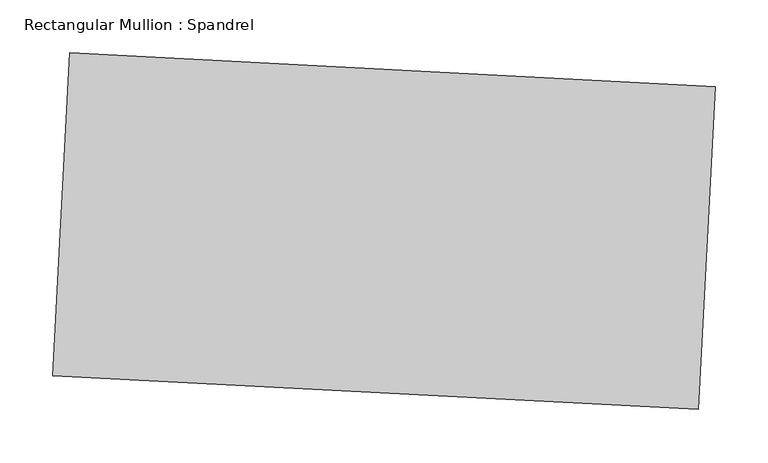
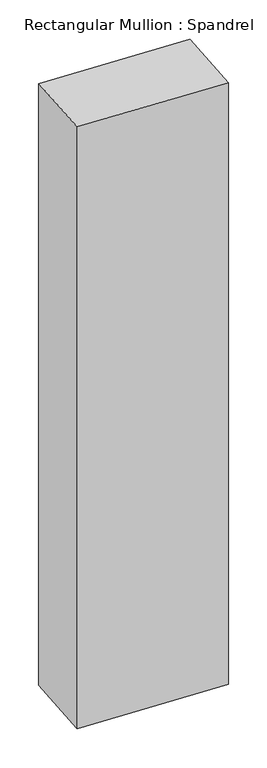
"""IFC4 building model written with IfcOpenShell, lengths in millimetres: member geometry, Rectangular Mullion : Spandrel."""

from ifc_helpers import new_model, si_unit, frame, origin, place, context, project, spatial, polyline, outline, extrude, source, transform, mapped, element, save


def rectangular_mullion_spandrel_46039ac9(model_context):
    return source(origin(), model_context, "Body", "SweptSolid", [
        extrude(outline(polyline([(312.3582819, 136.2391416), (296.4062825, -168.1431406), (-312.3582819, -136.2391416), (-296.4062825, 168.1431406), (312.3582819, 136.2391416)])), frame((0.0, 0.0, -2637.6144376), z_axis=(0.0, 0.0, 1.0), x_axis=(1.0, 0.0, 0.0)), (0.0, 0.0, 1.0), 2637.6144376),
    ])


if __name__ == "__main__":
    model = new_model("IFC4")
    model_context = context("Model", 3, world=origin())
    ifc_project = project(units=[si_unit("LENGTHUNIT", "METRE", prefix="MILLI")], contexts=[model_context])
    site = spatial("IfcSite", under=ifc_project)
    building = spatial("IfcBuilding", under=site)
    placement = place(None, origin())
    rectangular_mullion_spandrel_shape = rectangular_mullion_spandrel_46039ac9(model_context)
    element("IfcMember", 1, ObjectType="Rectangular Mullion : Spandrel", at=placement, inside=building, context=model_context, shape_type="MappedRepresentation", body=[
        mapped(rectangular_mullion_spandrel_shape, transform((0.0, 0.0, 0.0), x_axis=(1.0, 0.0, 0.0), y_axis=(0.0, 1.0, 0.0), z_axis=(0.0, 0.0, 1.0))),
    ])
    save(model, "model.ifc")

# Revit data of these elements
# Type "Rectangular Mullion : Spandrel"
#   built-in parameter 1007304 = 1 (stored number, unit not read)
#   built-in parameter 1007301 = 1 (stored number, unit not read)
#   built-in parameter 1007300 = 1 (stored number, unit not read)
# Element 1 (IfcMember, "Rectangular Mullion : Spandrel")
#   Materials on its faces: "Aluminum"
# Materials
#   "Aluminum": class "Metal", colour RGB 247 247 247, transparency 0, Description = "Aluminum 6061", Cost = 0
